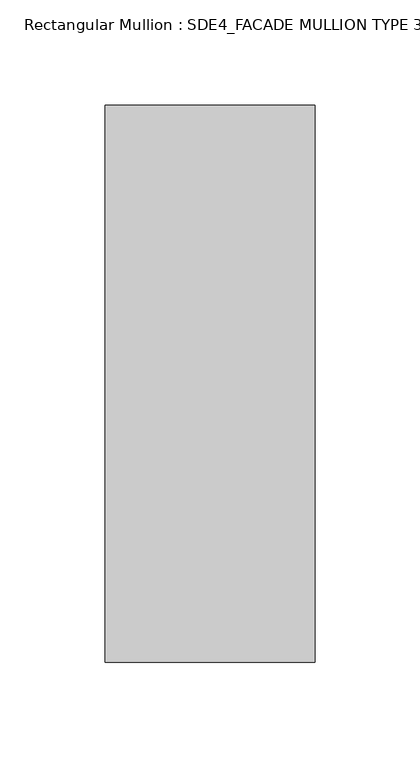
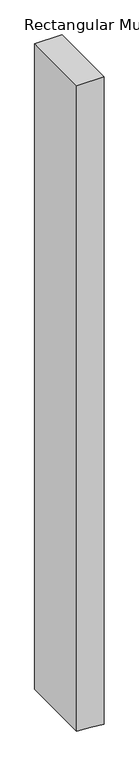
"""IFC4 building model written with IfcOpenShell, lengths in millimetres: member geometry, Rectangular Mullion : SDE4_FACADE MULLION TYPE 3."""

import ifcopenshell
import ifcopenshell.guid

model = None  # the IFC model being written
_history = None  # IfcOwnerHistory: only IFC2X3 demands one
_inside = {}  # id of a spatial element -> (the spatial element, [elements in it])
_under = {}  # id of a project, library or spatial element -> (it, [spatial elements below it])
_declared = {}  # id of a project -> (the project, [libraries it declares])
_typed = {}  # id of a type object -> (the type object, [elements of that type])
_made_of = {}  # id of a material, layer set ... -> (it, [elements and type objects made of it])


def new_model(schema):
    """Start an empty IFC model of exactly this schema.

    Asked for "IFC4X3", IfcOpenShell would pick the latest addendum, in which some entities
    have other attributes; the version numbers below select the first issue.
    IFC2X3 requires an IfcOwnerHistory on every rooted entity: one is made here for all.
    """
    global model, _history
    if schema == "IFC4X3":
        model = ifcopenshell.file(schema_version=(4, 3, 0, 0))
    else:
        model = ifcopenshell.file(schema=schema)
    _inside.clear()
    _under.clear()
    _declared.clear()
    _typed.clear()
    _made_of.clear()
    _history = None
    if model.schema == "IFC2X3":
        org = make("IfcOrganization", Name="unknown")
        user = make(
            "IfcPersonAndOrganization",
            ThePerson=make("IfcPerson", FamilyName="unknown"),
            TheOrganization=org,
        )
        app = make(
            "IfcApplication",
            ApplicationDeveloper=org,
            Version="unknown",
            ApplicationFullName="unknown",
            ApplicationIdentifier="unknown",
        )
        _history = make(
            "IfcOwnerHistory",
            OwningUser=user,
            OwningApplication=app,
            ChangeAction="ADDED",
            CreationDate=0,
        )
    return model


def make(cls, **values):
    """One entity of the class cls with the attributes given. An attribute that is None is left unset."""
    return model.create_entity(
        cls, **{name: value for name, value in values.items() if value is not None}
    )


def rooted(cls, **values):
    """An entity with a GlobalId (a new one), such as an element, a storey or a relation."""
    return make(cls, GlobalId=ifcopenshell.guid.new(), OwnerHistory=_history, **values)


def si_unit(unit_type, name, prefix=None):
    """IfcSIUnit, for example si_unit("LENGTHUNIT", "METRE", prefix="MILLI")."""
    return make("IfcSIUnit", UnitType=unit_type, Prefix=prefix, Name=name)


def assignment(units):
    """IfcUnitAssignment: the units of a project."""
    return None if units is None else make("IfcUnitAssignment", Units=units)


def point(xyz):
    """IfcCartesianPoint."""
    return None if xyz is None else make("IfcCartesianPoint", Coordinates=xyz)


def direction(xyz):
    """IfcDirection."""
    return None if xyz is None else make("IfcDirection", DirectionRatios=xyz)


def frame(location, z_axis=None, x_axis=None):
    """IfcAxis2Placement3D, a coordinate frame: its origin and axes. An axis left out is left unset."""
    return make(
        "IfcAxis2Placement3D",
        Location=point(location),
        Axis=direction(z_axis),
        RefDirection=direction(x_axis),
    )


def origin():
    """The frame at (0, 0, 0) with its axes left unset."""
    return frame((0.0, 0.0, 0.0))


def place(relative_to, where):
    """IfcLocalPlacement: puts the frame where relative to a parent placement (None: the world)."""
    return make(
        "IfcLocalPlacement", PlacementRelTo=relative_to, RelativePlacement=where
    )


def context(
    kind, dimensions, precision=None, world=None, true_north=None, identifier=None
):
    """IfcGeometricRepresentationContext, for example the 3D "Model" context."""
    return make(
        "IfcGeometricRepresentationContext",
        ContextIdentifier=identifier,
        ContextType=kind,
        CoordinateSpaceDimension=dimensions,
        Precision=precision,
        WorldCoordinateSystem=world,
        TrueNorth=true_north,
    )


def project(units=None, contexts=None):
    """IfcProject with its units and contexts."""
    return rooted(
        "IfcProject",
        Name="project",
        RepresentationContexts=contexts,
        UnitsInContext=assignment(units),
    )


def spatial(cls, under=None, at=None, **own):
    """A site, building, storey or space (cls), placed at a placement, below another one or the project."""
    s = rooted(cls, ObjectPlacement=at, **own)
    if under is not None:
        _under.setdefault(under.id(), (under, []))[1].append(s)
    return s


def polyline(points):
    """IfcPolyline through the points."""
    return make("IfcPolyline", Points=[point(p) for p in points])


def outline(outer, holes=None, kind="AREA"):
    """IfcArbitraryClosedProfileDef: a profile drawn as a closed curve; with holes, ...WithVoids."""
    if holes is None:
        return make("IfcArbitraryClosedProfileDef", ProfileType=kind, OuterCurve=outer)
    return make(
        "IfcArbitraryProfileDefWithVoids",
        ProfileType=kind,
        OuterCurve=outer,
        InnerCurves=holes,
    )


def extrude(swept, where, along, depth):
    """IfcExtrudedAreaSolid: the profile swept, set in the frame where, extruded along a direction by depth."""
    return make(
        "IfcExtrudedAreaSolid",
        SweptArea=swept,
        Position=where,
        ExtrudedDirection=direction(along),
        Depth=depth,
    )


def shape(context_of_items, identifier, shape_type, items):
    """IfcShapeRepresentation: the items that make up one representation, for example the "Body"."""
    return make(
        "IfcShapeRepresentation",
        ContextOfItems=context_of_items,
        RepresentationIdentifier=identifier,
        RepresentationType=shape_type,
        Items=items,
    )


def source(mapping_origin, context_of_items, identifier, shape_type, items):
    """IfcRepresentationMap: a shape defined once, which mapped items show again and again."""
    return make(
        "IfcRepresentationMap",
        MappingOrigin=mapping_origin,
        MappedRepresentation=shape(context_of_items, identifier, shape_type, items),
    )


def transform(
    local_origin,
    x_axis=None,
    y_axis=None,
    z_axis=None,
    scale=None,
    scale2=None,
    scale3=None,
    uniform=True,
):
    """IfcCartesianTransformationOperator3D, or its non-uniform kind. x_axis, y_axis, z_axis: its Axis1, 2, 3."""
    if uniform:
        return make(
            "IfcCartesianTransformationOperator3D",
            Axis1=direction(x_axis),
            Axis2=direction(y_axis),
            LocalOrigin=point(local_origin),
            Scale=scale,
            Axis3=direction(z_axis),
        )
    return make(
        "IfcCartesianTransformationOperator3DnonUniform",
        Axis1=direction(x_axis),
        Axis2=direction(y_axis),
        LocalOrigin=point(local_origin),
        Scale=scale,
        Axis3=direction(z_axis),
        Scale2=scale2,
        Scale3=scale3,
    )


def mapped(mapping_source, mapping_target):
    """IfcMappedItem: shows the shape of a source again, moved by a transform."""
    return make(
        "IfcMappedItem", MappingSource=mapping_source, MappingTarget=mapping_target
    )


def made_of(thing, what):
    """Note that an element or type object is made of a material, layer set ...; save() writes the relation."""
    if what is not None:
        _made_of.setdefault(what.id(), (what, []))[1].append(thing)
    return thing


def element(
    cls,
    number,
    at=None,
    inside=None,
    cuts=None,
    type_object=None,
    material=None,
    context=None,
    identifier="Body",
    shape_type=None,
    held_by="IfcProductDefinitionShape",
    body=None,
    shapes=None,
    **own,
):
    """One element of the class cls, such as IfcWall. Its Tag is "e" and its number.

    at: its placement. inside: the storey or other place that contains it. cuts: it is an
    opening in that element (IfcRelVoidsElement). A single representation is given by context,
    identifier, shape_type and body (its items); several are given by shapes. held_by: the class
    of the entity that holds the representations. save() writes the other relations.
    """
    e = rooted(cls, Tag="e%d" % number, ObjectPlacement=at, **own)
    if body is not None:
        shapes = [shape(context, identifier, shape_type, body)]
    if shapes is not None:
        e.Representation = make(held_by, Representations=shapes)
    if inside is not None:
        _inside.setdefault(inside.id(), (inside, []))[1].append(e)
    if cuts is not None:
        rooted(
            "IfcRelVoidsElement", RelatingBuildingElement=cuts, RelatedOpeningElement=e
        )
    if type_object is not None:
        _typed.setdefault(type_object.id(), (type_object, []))[1].append(e)
    return made_of(e, material)


def aggregate(whole, parts):
    """IfcRelAggregates: a whole, such as a stair, and the parts it consists of."""
    return rooted("IfcRelAggregates", RelatingObject=whole, RelatedObjects=parts)


def save(model, path):
    """Write the relations noted so far, then the file.

    IfcRelAggregates (storeys below a building ...), IfcRelContainedInSpatialStructure (elements
    in a storey), IfcRelDefinesByType, IfcRelAssociatesMaterial and IfcRelDeclares: one each for
    every whole, place, type object, material and project.
    """
    for whole, parts in _under.values():
        aggregate(whole, parts)
    for where, things in _inside.values():
        rooted(
            "IfcRelContainedInSpatialStructure",
            RelatedElements=things,
            RelatingStructure=where,
        )
    for kind, things in _typed.values():
        rooted("IfcRelDefinesByType", RelatedObjects=things, RelatingType=kind)
    for what, things in _made_of.values():
        rooted("IfcRelAssociatesMaterial", RelatedObjects=things, RelatingMaterial=what)
    for by, libraries in _declared.values():
        rooted("IfcRelDeclares", RelatingContext=by, RelatedDefinitions=libraries)
    model.write(path)


def rectangular_mullion_sde4_facade_mullion_type_3_74c64f3e(model_context):
    return source(origin(), model_context, "Body", "SweptSolid", [
        extrude(outline(polyline([(0.0, 50.0), (0.0, -50.0), (-2487.3759917, -50.0), (-2491.4420707, 3.056508), (-2495.039668, 50.0), (0.0, 50.0)])), frame((0.0, -132.5, 0.0), z_axis=(0.0, 1.0, 0.0), x_axis=(0.0, 0.0, 1.0)), (0.0, 0.0, 1.0), 265.0),
    ])


if __name__ == "__main__":
    model = new_model("IFC4")
    model_context = context("Model", 3, world=origin())
    ifc_project = project(units=[si_unit("LENGTHUNIT", "METRE", prefix="MILLI")], contexts=[model_context])
    site = spatial("IfcSite", under=ifc_project)
    building = spatial("IfcBuilding", under=site)
    placement = place(None, origin())
    rectangular_mullion_sde4_facade_mullion_type_3_shape = rectangular_mullion_sde4_facade_mullion_type_3_74c64f3e(model_context)
    element("IfcMember", 1, ObjectType="Rectangular Mullion : SDE4_FACADE MULLION TYPE 3", at=placement, inside=building, context=model_context, shape_type="MappedRepresentation", body=[
        mapped(rectangular_mullion_sde4_facade_mullion_type_3_shape, transform((0.0, 0.0, 0.0), x_axis=(1.0, 0.0, 0.0), y_axis=(0.0, 1.0, 0.0), z_axis=(0.0, 0.0, 1.0))),
    ])
    save(model, "model.ifc")

# Revit data of these elements
# Type "Rectangular Mullion : SDE4_FACADE MULLION TYPE 3"
#   built-in parameter 1007322 = 0.869423 (stored number, unit not read)
#   built-in parameter 1007321 = 0.164042 (stored number, unit not read)
#   built-in parameter 1007320 = 0.164042 (stored number, unit not read)
